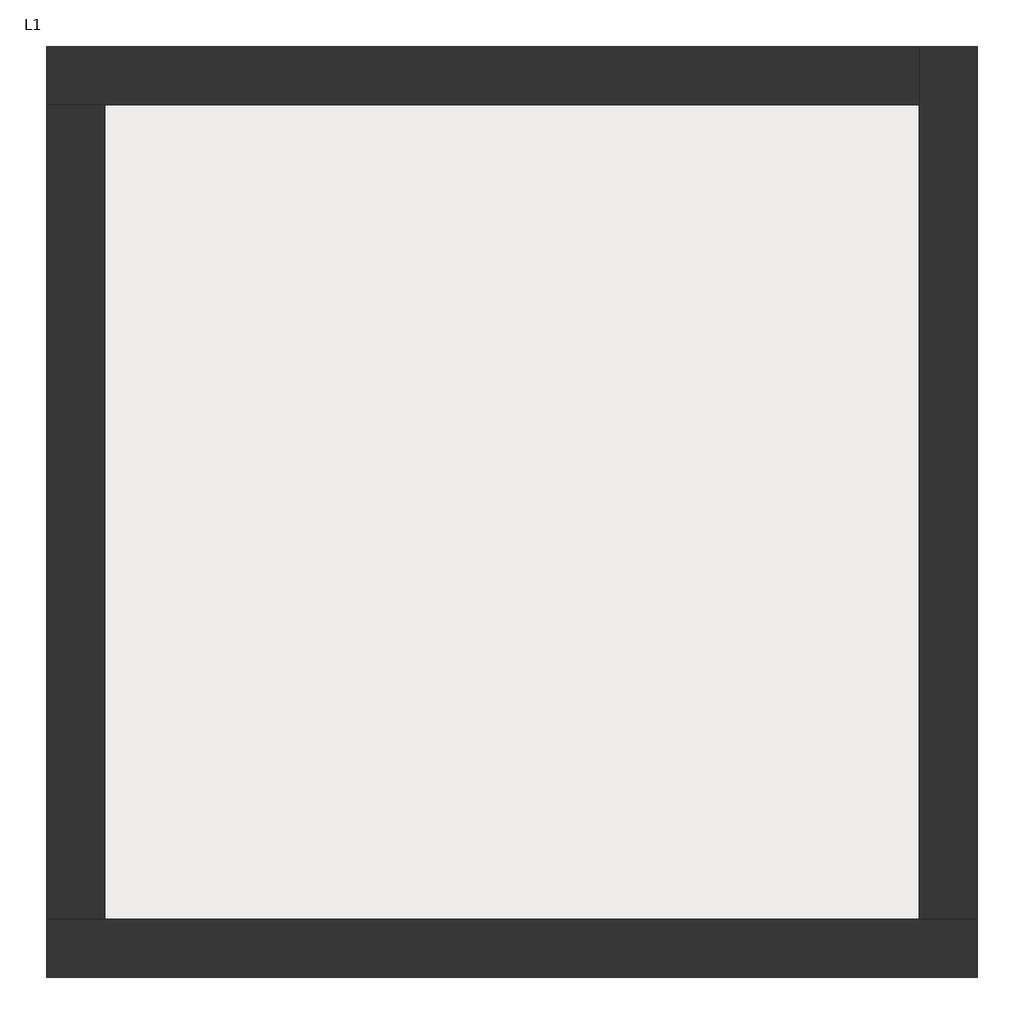
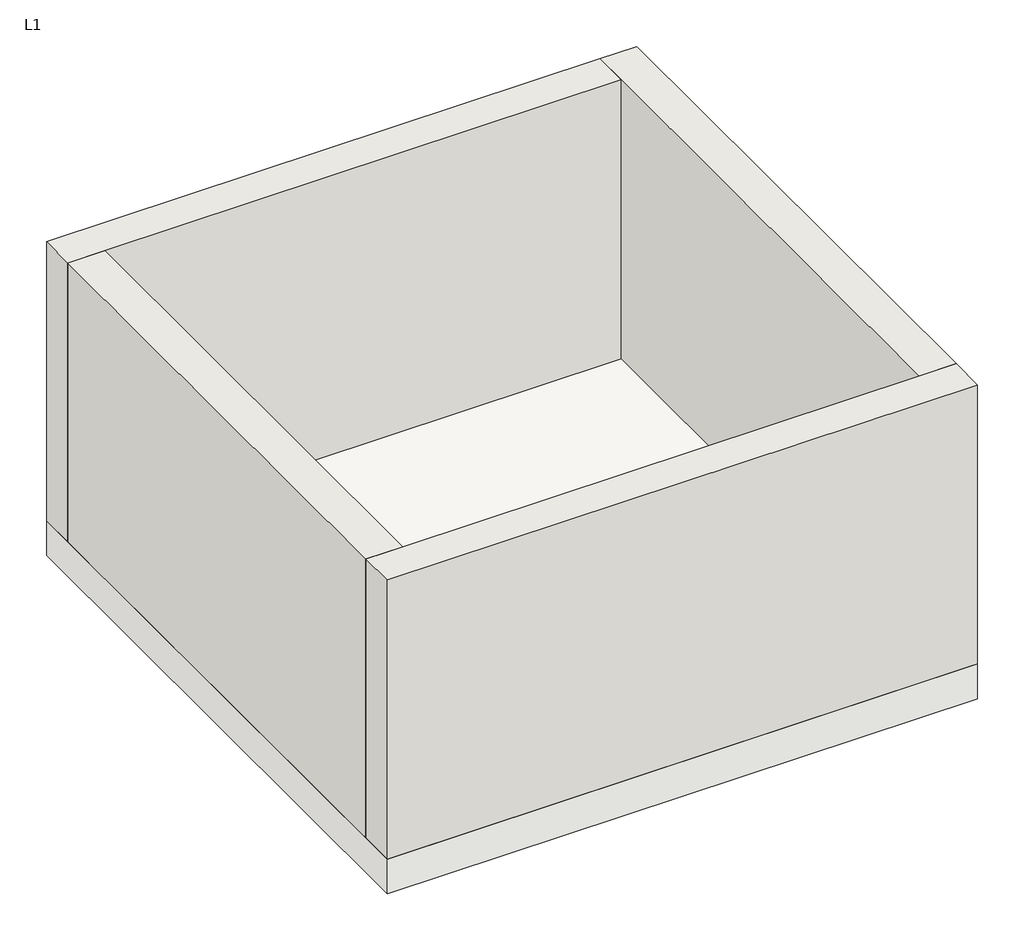
# One storey: 4 walls, 1 slab.
"""IFC4 building model written with IfcOpenShell, lengths in millimetres."""

from ifc_helpers import new_model, si_unit, frame, origin, origin_with_axes, place, context, project, spatial, polyline, outline, extrude, faceted_brep, element, save

model = new_model("IFC4")

# Units and contexts
model_context = context("Model", 3, world=origin())
ifc_project = project(units=[si_unit("LENGTHUNIT", "METRE", prefix="MILLI")], contexts=[model_context])

# Site, building, storey
site = spatial("IfcSite", under=ifc_project)
building = spatial("IfcBuilding", under=site)
storey = spatial("IfcBuildingStorey", under=building, Name="L1", Elevation=0.0)

# Slab
placement = place(None, origin())
element("IfcSlab", 1, ObjectType="FOR INT AC-NH", at=placement, inside=storey, context=model_context, shape_type="SweptSolid", body=[
    extrude(outline(polyline([(0.0, 7999.99416), (7999.99416, 7999.99416), (7999.99416, 0.0), (0.0, 0.0), (0.0, 7999.99416)])), frame((0.0, 0.0, -499.9999972), z_axis=(0.0, 0.0, 1.0), x_axis=(1.0, 0.0, 0.0)), (0.0, 0.0, 1.0), 499.9999972),
])

# Walls
element("IfcWall", 2, ObjectType="MURO EXTERIOR0.60", at=placement, inside=storey, context=model_context, shape_type="Brep", body=[
    faceted_brep([(0.0, 0.0, 0.0), (7999.99416, 0.0, 0.0), (7999.99416, 0.0, 4000.01232), (0.0, 0.0, 4000.01232), (0.0, 500.000016, 0.0), (0.0, 500.000016, 4000.01232), (500.000016, 500.000016, 4000.01232), (7499.994144, 500.000016, 4000.01232), (7999.99416, 500.000016, 4000.01232), (7999.99416, 500.000016, 0.0), (7499.994144, 500.000016, 0.0), (500.000016, 500.000016, 0.0)], [[[0, 1, 2, 3]], [[4, 5, 6, 7, 8, 9, 10, 11]], [[1, 0, 4, 11, 10, 9]], [[3, 2, 8, 7, 6, 5]], [[2, 1, 9, 8]], [[0, 3, 5, 4]]]),
])
element("IfcWall", 3, ObjectType="MURO EXTERIOR0.60", at=placement, inside=storey, context=model_context, shape_type="Brep", body=[
    faceted_brep([(7999.99416, 500.000016, 0.0), (7999.99416, 7999.99416, 0.0), (7999.99416, 7999.99416, 4000.01232), (7999.99416, 500.000016, 4000.01232), (7499.994144, 500.000016, 0.0), (7499.994144, 500.000016, 4000.01232), (7499.994144, 7499.994144, 4000.01232), (7499.994144, 7999.99416, 4000.01232), (7499.994144, 7999.99416, 0.0), (7499.994144, 7499.994144, 0.0)], [[[0, 1, 2, 3]], [[4, 5, 6, 7, 8, 9]], [[1, 0, 4, 9, 8]], [[3, 2, 7, 6, 5]], [[2, 1, 8, 7]], [[0, 3, 5, 4]]]),
])
element("IfcWall", 4, ObjectType="MURO EXTERIOR0.60", at=placement, inside=storey, context=model_context, shape_type="Brep", body=[
    faceted_brep([(7499.994144, 7999.99416, 0.0), (0.0, 7999.99416, 0.0), (0.0, 7999.99416, 4000.01232), (7499.994144, 7999.99416, 4000.01232), (7499.994144, 7499.994144, 0.0), (7499.994144, 7499.994144, 4000.01232), (500.000016, 7499.994144, 4000.01232), (0.0, 7499.994144, 4000.01232), (0.0, 7499.994144, 0.0), (500.000016, 7499.994144, 0.0)], [[[0, 1, 2, 3]], [[4, 5, 6, 7, 8, 9]], [[1, 0, 4, 9, 8]], [[3, 2, 7, 6, 5]], [[2, 1, 8, 7]], [[0, 3, 5, 4]]]),
])
element("IfcWall", 5, ObjectType="MURO EXTERIOR0.60", at=placement, inside=storey, context=model_context, shape_type="SweptSolid", body=[
    extrude(outline(polyline([(0.0, 500.000016), (0.0, 7499.994144), (500.000016, 7499.994144), (500.000016, 500.000016), (0.0, 500.000016)])), origin_with_axes(), (0.0, 0.0, 1.0), 4000.01232),
])

save(model, "model.ifc")

# Revit data of these elements
# Type "FOR INT AC-NH"
#   Layers, outside or top first: 0.010 m "Plaqueta o baldosa de gres" (function 1); 0.055 m "Mortero de cemento o cal para albañilería y para revoco-enlucido d entre 1000 y 1250" (function 1); 0.120 m "Poliestireno Expandido XPS" (function 1); 0.250 m "FU Entrevigado cerámico -Canto 250 mm" (function 1); 0.050 m "Cámara de aire sin ventilar horizontal 5 cm" (function 1); 0.015 m "Placa de yeso laminado (PYL) d entre 750 y 900" (function 1)
# Type "MURO EXTERIOR0.60"
#   Description = "Metal Studs with Brick over sheathing on exterior and Gypsum Wall Board (GWB) on interior, Exterior Function"
#   Assembly Code = "B2010158"
#   Type Mark = "W10"
#   Layers, outside or top first: 0.030 m no material (function 1); 0.140 m no material (function 1); 0.240 m no material (function 1); 0.010 m no material (function 1); 0.050 m no material (function 1); 0.015 m no material (function 1); 0.015 m no material (function 1)
# Element 1 (IfcSlab, "FOR INT AC-NH")
#   Height Offset From Level = 0.000 m
#   Phase Created = New Construction
#   Materials on its faces: "Placa de yeso laminado (PYL) d entre 750 y 900", "Plaqueta o baldosa de gres"
# Elements 2, 3, 4, 5 (IfcWall, "MURO EXTERIOR0.60")
#   Top Offset = 0.000 m
#   Base Offset = 0.000 m
#   Unconnected Height = 4.000012 m
#   wall height = 4.000012 m
#   Phase Created = New Construction
#   Base Constraint = L1
#   Materials on its faces: "Default Wall"
# Materials
#   "Plaqueta o baldosa de gres": class "Cerámicos", colour RGB 0 0 0, transparency 0, Comments = "CTE"
#   "Mortero de cemento o cal para albañilería y para revoco-enlucido d entre 1000 y 1250": class "Morteros", colour RGB 0 0 0, transparency 0, Comments = "CTE"
#   "Poliestireno Expandido XPS": class "Plásticos", colour RGB 0 0 0, transparency 0, Comments = "CTE"
#   "FU Entrevigado cerámico -Canto 250 mm": class "Forjados unidireccionales", colour RGB 0 0 0, transparency 0, Comments = "CTE"
#   "Cámara de aire sin ventilar horizontal 5 cm": class "Cámaras de aire", colour RGB 0 0 0, transparency 0, Comments = "CTE"
#   "Placa de yeso laminado (PYL) d entre 750 y 900": class "Yesos", colour RGB 0 0 0, transparency 0, Comments = "CTE"
#   "Default Wall": class "Miscellaneous", colour RGB 192 192 192, transparency 0, Cost = 0
